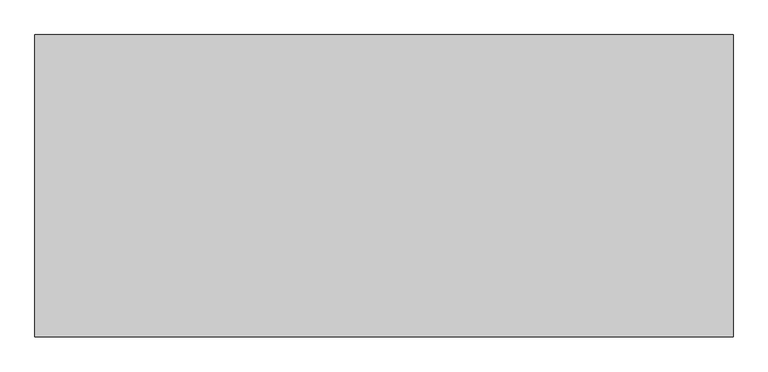
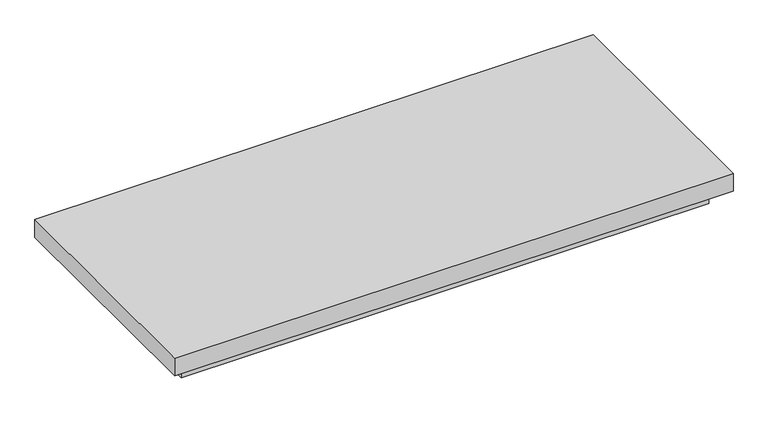
"""IFC4 building model written with IfcOpenShell, lengths in millimetres: proxy geometry, TAMPO - CASA DE MÁQUINA : TAMPO - CASA DE MÁQUINA."""

import ifcopenshell
import ifcopenshell.guid

model = None  # the IFC model being written
_history = None  # IfcOwnerHistory: only IFC2X3 demands one
_inside = {}  # id of a spatial element -> (the spatial element, [elements in it])
_under = {}  # id of a project, library or spatial element -> (it, [spatial elements below it])
_declared = {}  # id of a project -> (the project, [libraries it declares])
_typed = {}  # id of a type object -> (the type object, [elements of that type])
_made_of = {}  # id of a material, layer set ... -> (it, [elements and type objects made of it])


def new_model(schema):
    """Start an empty IFC model of exactly this schema.

    Asked for "IFC4X3", IfcOpenShell would pick the latest addendum, in which some entities
    have other attributes; the version numbers below select the first issue.
    IFC2X3 requires an IfcOwnerHistory on every rooted entity: one is made here for all.
    """
    global model, _history
    if schema == "IFC4X3":
        model = ifcopenshell.file(schema_version=(4, 3, 0, 0))
    else:
        model = ifcopenshell.file(schema=schema)
    _inside.clear()
    _under.clear()
    _declared.clear()
    _typed.clear()
    _made_of.clear()
    _history = None
    if model.schema == "IFC2X3":
        org = make("IfcOrganization", Name="unknown")
        user = make(
            "IfcPersonAndOrganization",
            ThePerson=make("IfcPerson", FamilyName="unknown"),
            TheOrganization=org,
        )
        app = make(
            "IfcApplication",
            ApplicationDeveloper=org,
            Version="unknown",
            ApplicationFullName="unknown",
            ApplicationIdentifier="unknown",
        )
        _history = make(
            "IfcOwnerHistory",
            OwningUser=user,
            OwningApplication=app,
            ChangeAction="ADDED",
            CreationDate=0,
        )
    return model


def make(cls, **values):
    """One entity of the class cls with the attributes given. An attribute that is None is left unset."""
    return model.create_entity(
        cls, **{name: value for name, value in values.items() if value is not None}
    )


def rooted(cls, **values):
    """An entity with a GlobalId (a new one), such as an element, a storey or a relation."""
    return make(cls, GlobalId=ifcopenshell.guid.new(), OwnerHistory=_history, **values)


def si_unit(unit_type, name, prefix=None):
    """IfcSIUnit, for example si_unit("LENGTHUNIT", "METRE", prefix="MILLI")."""
    return make("IfcSIUnit", UnitType=unit_type, Prefix=prefix, Name=name)


def assignment(units):
    """IfcUnitAssignment: the units of a project."""
    return None if units is None else make("IfcUnitAssignment", Units=units)


def point(xyz):
    """IfcCartesianPoint."""
    return None if xyz is None else make("IfcCartesianPoint", Coordinates=xyz)


def direction(xyz):
    """IfcDirection."""
    return None if xyz is None else make("IfcDirection", DirectionRatios=xyz)


def frame(location, z_axis=None, x_axis=None):
    """IfcAxis2Placement3D, a coordinate frame: its origin and axes. An axis left out is left unset."""
    return make(
        "IfcAxis2Placement3D",
        Location=point(location),
        Axis=direction(z_axis),
        RefDirection=direction(x_axis),
    )


def origin():
    """The frame at (0, 0, 0) with its axes left unset."""
    return frame((0.0, 0.0, 0.0))


def place(relative_to, where):
    """IfcLocalPlacement: puts the frame where relative to a parent placement (None: the world)."""
    return make(
        "IfcLocalPlacement", PlacementRelTo=relative_to, RelativePlacement=where
    )


def context(
    kind, dimensions, precision=None, world=None, true_north=None, identifier=None
):
    """IfcGeometricRepresentationContext, for example the 3D "Model" context."""
    return make(
        "IfcGeometricRepresentationContext",
        ContextIdentifier=identifier,
        ContextType=kind,
        CoordinateSpaceDimension=dimensions,
        Precision=precision,
        WorldCoordinateSystem=world,
        TrueNorth=true_north,
    )


def project(units=None, contexts=None):
    """IfcProject with its units and contexts."""
    return rooted(
        "IfcProject",
        Name="project",
        RepresentationContexts=contexts,
        UnitsInContext=assignment(units),
    )


def spatial(cls, under=None, at=None, **own):
    """A site, building, storey or space (cls), placed at a placement, below another one or the project."""
    s = rooted(cls, ObjectPlacement=at, **own)
    if under is not None:
        _under.setdefault(under.id(), (under, []))[1].append(s)
    return s


def polyline(points):
    """IfcPolyline through the points."""
    return make("IfcPolyline", Points=[point(p) for p in points])


def outline(outer, holes=None, kind="AREA"):
    """IfcArbitraryClosedProfileDef: a profile drawn as a closed curve; with holes, ...WithVoids."""
    if holes is None:
        return make("IfcArbitraryClosedProfileDef", ProfileType=kind, OuterCurve=outer)
    return make(
        "IfcArbitraryProfileDefWithVoids",
        ProfileType=kind,
        OuterCurve=outer,
        InnerCurves=holes,
    )


def extrude(swept, where, along, depth):
    """IfcExtrudedAreaSolid: the profile swept, set in the frame where, extruded along a direction by depth."""
    return make(
        "IfcExtrudedAreaSolid",
        SweptArea=swept,
        Position=where,
        ExtrudedDirection=direction(along),
        Depth=depth,
    )


def shape(context_of_items, identifier, shape_type, items):
    """IfcShapeRepresentation: the items that make up one representation, for example the "Body"."""
    return make(
        "IfcShapeRepresentation",
        ContextOfItems=context_of_items,
        RepresentationIdentifier=identifier,
        RepresentationType=shape_type,
        Items=items,
    )


def source(mapping_origin, context_of_items, identifier, shape_type, items):
    """IfcRepresentationMap: a shape defined once, which mapped items show again and again."""
    return make(
        "IfcRepresentationMap",
        MappingOrigin=mapping_origin,
        MappedRepresentation=shape(context_of_items, identifier, shape_type, items),
    )


def transform(
    local_origin,
    x_axis=None,
    y_axis=None,
    z_axis=None,
    scale=None,
    scale2=None,
    scale3=None,
    uniform=True,
):
    """IfcCartesianTransformationOperator3D, or its non-uniform kind. x_axis, y_axis, z_axis: its Axis1, 2, 3."""
    if uniform:
        return make(
            "IfcCartesianTransformationOperator3D",
            Axis1=direction(x_axis),
            Axis2=direction(y_axis),
            LocalOrigin=point(local_origin),
            Scale=scale,
            Axis3=direction(z_axis),
        )
    return make(
        "IfcCartesianTransformationOperator3DnonUniform",
        Axis1=direction(x_axis),
        Axis2=direction(y_axis),
        LocalOrigin=point(local_origin),
        Scale=scale,
        Axis3=direction(z_axis),
        Scale2=scale2,
        Scale3=scale3,
    )


def mapped(mapping_source, mapping_target):
    """IfcMappedItem: shows the shape of a source again, moved by a transform."""
    return make(
        "IfcMappedItem", MappingSource=mapping_source, MappingTarget=mapping_target
    )


def made_of(thing, what):
    """Note that an element or type object is made of a material, layer set ...; save() writes the relation."""
    if what is not None:
        _made_of.setdefault(what.id(), (what, []))[1].append(thing)
    return thing


def element(
    cls,
    number,
    at=None,
    inside=None,
    cuts=None,
    type_object=None,
    material=None,
    context=None,
    identifier="Body",
    shape_type=None,
    held_by="IfcProductDefinitionShape",
    body=None,
    shapes=None,
    **own,
):
    """One element of the class cls, such as IfcWall. Its Tag is "e" and its number.

    at: its placement. inside: the storey or other place that contains it. cuts: it is an
    opening in that element (IfcRelVoidsElement). A single representation is given by context,
    identifier, shape_type and body (its items); several are given by shapes. held_by: the class
    of the entity that holds the representations. save() writes the other relations.
    """
    e = rooted(cls, Tag="e%d" % number, ObjectPlacement=at, **own)
    if body is not None:
        shapes = [shape(context, identifier, shape_type, body)]
    if shapes is not None:
        e.Representation = make(held_by, Representations=shapes)
    if inside is not None:
        _inside.setdefault(inside.id(), (inside, []))[1].append(e)
    if cuts is not None:
        rooted(
            "IfcRelVoidsElement", RelatingBuildingElement=cuts, RelatedOpeningElement=e
        )
    if type_object is not None:
        _typed.setdefault(type_object.id(), (type_object, []))[1].append(e)
    return made_of(e, material)


def aggregate(whole, parts):
    """IfcRelAggregates: a whole, such as a stair, and the parts it consists of."""
    return rooted("IfcRelAggregates", RelatingObject=whole, RelatedObjects=parts)


def save(model, path):
    """Write the relations noted so far, then the file.

    IfcRelAggregates (storeys below a building ...), IfcRelContainedInSpatialStructure (elements
    in a storey), IfcRelDefinesByType, IfcRelAssociatesMaterial and IfcRelDeclares: one each for
    every whole, place, type object, material and project.
    """
    for whole, parts in _under.values():
        aggregate(whole, parts)
    for where, things in _inside.values():
        rooted(
            "IfcRelContainedInSpatialStructure",
            RelatedElements=things,
            RelatingStructure=where,
        )
    for kind, things in _typed.values():
        rooted("IfcRelDefinesByType", RelatedObjects=things, RelatingType=kind)
    for what, things in _made_of.values():
        rooted("IfcRelAssociatesMaterial", RelatedObjects=things, RelatingMaterial=what)
    for by, libraries in _declared.values():
        rooted("IfcRelDeclares", RelatingContext=by, RelatedDefinitions=libraries)
    model.write(path)


def specialty_equipment_67e2e29c(model_context):
    return source(origin(), model_context, "Body", "SweptSolid", [
        extrude(outline(polyline([(12687.718693, 5627.4300153), (12687.718693, 4481.4300153), (10041.718693, 4481.4300153), (10041.718693, 5627.4300153), (12687.718693, 5627.4300153)])), frame((0.0, 0.0, 280.0), z_axis=(0.0, 0.0, 1.0), x_axis=(1.0, 0.0, 0.0)), (0.0, 0.0, 1.0), 88.4706632),
        extrude(outline(polyline([(12614.718693, 5554.4300153), (12614.718693, 4554.4300153), (10114.718693, 4554.4300153), (10114.718693, 5554.4300153), (12614.718693, 5554.4300153)])), frame((0.0, 0.0, 200.0), z_axis=(0.0, 0.0, 1.0), x_axis=(1.0, 0.0, 0.0)), (0.0, 0.0, 1.0), 80.0),
    ])


if __name__ == "__main__":
    model = new_model("IFC4")
    model_context = context("Model", 3, world=origin())
    ifc_project = project(units=[si_unit("LENGTHUNIT", "METRE", prefix="MILLI")], contexts=[model_context])
    site = spatial("IfcSite", under=ifc_project)
    building = spatial("IfcBuilding", under=site)
    placement = place(None, origin())
    specialty_equipment_shape = specialty_equipment_67e2e29c(model_context)
    element("IfcBuildingElementProxy", 1, Name="TAMPO - CASA DE MÁQUINA : TAMPO - CASA DE MÁQUINA", ObjectType="TAMPO - CASA DE MÁQUINA : TAMPO - CASA DE MÁQUINA", at=placement, inside=building, context=model_context, shape_type="MappedRepresentation", body=[
        mapped(specialty_equipment_shape, transform((0.0, 0.0, 0.0), x_axis=(1.0, 0.0, 0.0), y_axis=(0.0, 1.0, 0.0), z_axis=(0.0, 0.0, 1.0))),
    ])
    save(model, "model.ifc")

# Revit data of these elements
# Element 1 (IfcBuildingElementProxy, "TAMPO - CASA DE MÁQUINA : TAMPO - CASA DE MÁQUINA")
#   Materials on its faces: ".ALUMÍNIO"
# Materials
#   ".ALUMÍNIO": class "CC_METAIS", colour RGB 244 244 244, transparency 0, Description = "Material alumínio", Cost = 0
